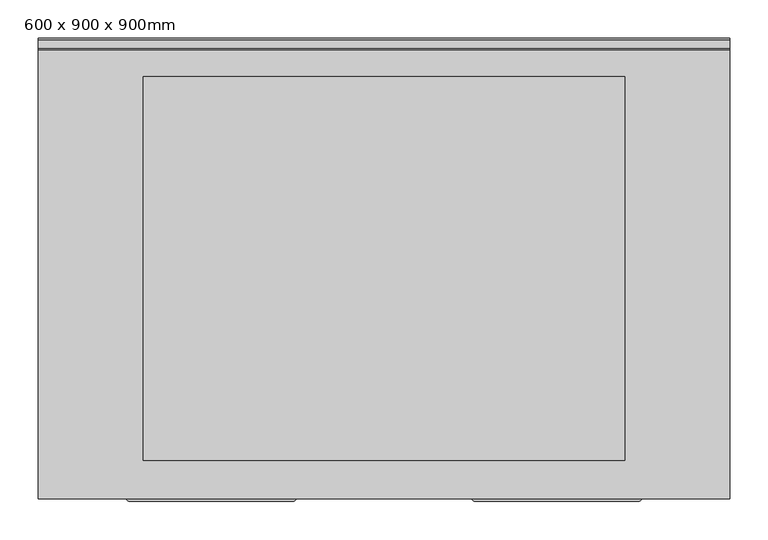
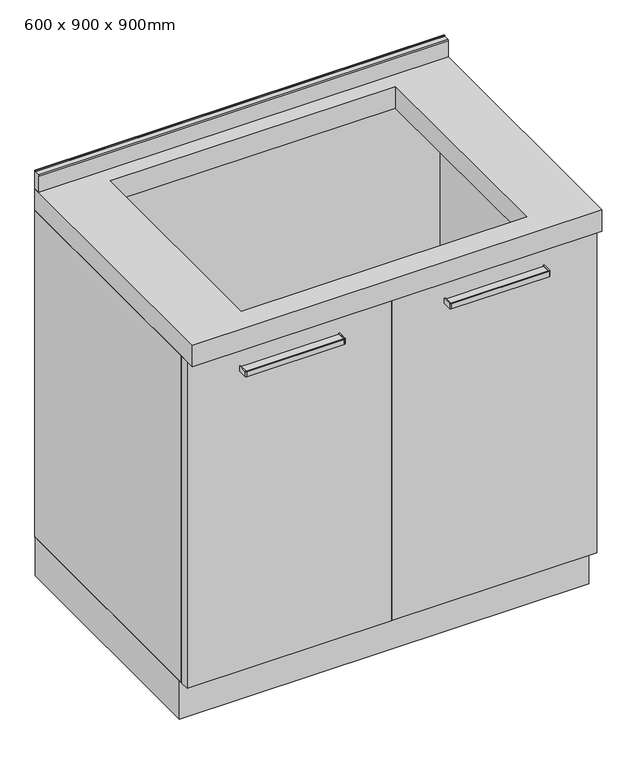
"""IFC4 building model written with IfcOpenShell, lengths in millimetres: furniture geometry, Küchenelement (1) - 2-flg - für Spüle : 600 x 900 x 900mm."""

import ifcopenshell
import ifcopenshell.guid

model = None  # the IFC model being written
_history = None  # IfcOwnerHistory: only IFC2X3 demands one
_inside = {}  # id of a spatial element -> (the spatial element, [elements in it])
_under = {}  # id of a project, library or spatial element -> (it, [spatial elements below it])
_declared = {}  # id of a project -> (the project, [libraries it declares])
_typed = {}  # id of a type object -> (the type object, [elements of that type])
_made_of = {}  # id of a material, layer set ... -> (it, [elements and type objects made of it])


def new_model(schema):
    """Start an empty IFC model of exactly this schema.

    Asked for "IFC4X3", IfcOpenShell would pick the latest addendum, in which some entities
    have other attributes; the version numbers below select the first issue.
    IFC2X3 requires an IfcOwnerHistory on every rooted entity: one is made here for all.
    """
    global model, _history
    if schema == "IFC4X3":
        model = ifcopenshell.file(schema_version=(4, 3, 0, 0))
    else:
        model = ifcopenshell.file(schema=schema)
    _inside.clear()
    _under.clear()
    _declared.clear()
    _typed.clear()
    _made_of.clear()
    _history = None
    if model.schema == "IFC2X3":
        org = make("IfcOrganization", Name="unknown")
        user = make(
            "IfcPersonAndOrganization",
            ThePerson=make("IfcPerson", FamilyName="unknown"),
            TheOrganization=org,
        )
        app = make(
            "IfcApplication",
            ApplicationDeveloper=org,
            Version="unknown",
            ApplicationFullName="unknown",
            ApplicationIdentifier="unknown",
        )
        _history = make(
            "IfcOwnerHistory",
            OwningUser=user,
            OwningApplication=app,
            ChangeAction="ADDED",
            CreationDate=0,
        )
    return model


def make(cls, **values):
    """One entity of the class cls with the attributes given. An attribute that is None is left unset."""
    return model.create_entity(
        cls, **{name: value for name, value in values.items() if value is not None}
    )


def rooted(cls, **values):
    """An entity with a GlobalId (a new one), such as an element, a storey or a relation."""
    return make(cls, GlobalId=ifcopenshell.guid.new(), OwnerHistory=_history, **values)


def si_unit(unit_type, name, prefix=None):
    """IfcSIUnit, for example si_unit("LENGTHUNIT", "METRE", prefix="MILLI")."""
    return make("IfcSIUnit", UnitType=unit_type, Prefix=prefix, Name=name)


def assignment(units):
    """IfcUnitAssignment: the units of a project."""
    return None if units is None else make("IfcUnitAssignment", Units=units)


def point(xyz):
    """IfcCartesianPoint."""
    return None if xyz is None else make("IfcCartesianPoint", Coordinates=xyz)


def direction(xyz):
    """IfcDirection."""
    return None if xyz is None else make("IfcDirection", DirectionRatios=xyz)


def frame(location, z_axis=None, x_axis=None):
    """IfcAxis2Placement3D, a coordinate frame: its origin and axes. An axis left out is left unset."""
    return make(
        "IfcAxis2Placement3D",
        Location=point(location),
        Axis=direction(z_axis),
        RefDirection=direction(x_axis),
    )


def frame_2d(location, x_axis=None):
    """IfcAxis2Placement2D, a coordinate frame in the plane: its origin and x axis."""
    return make(
        "IfcAxis2Placement2D", Location=point(location), RefDirection=direction(x_axis)
    )


def origin():
    """The frame at (0, 0, 0) with its axes left unset."""
    return frame((0.0, 0.0, 0.0))


def origin_with_axes():
    """The frame at (0, 0, 0) with the z axis (0, 0, 1) and the x axis (1, 0, 0) written out."""
    return frame((0.0, 0.0, 0.0), z_axis=(0.0, 0.0, 1.0), x_axis=(1.0, 0.0, 0.0))


def place(relative_to, where):
    """IfcLocalPlacement: puts the frame where relative to a parent placement (None: the world)."""
    return make(
        "IfcLocalPlacement", PlacementRelTo=relative_to, RelativePlacement=where
    )


def context(
    kind, dimensions, precision=None, world=None, true_north=None, identifier=None
):
    """IfcGeometricRepresentationContext, for example the 3D "Model" context."""
    return make(
        "IfcGeometricRepresentationContext",
        ContextIdentifier=identifier,
        ContextType=kind,
        CoordinateSpaceDimension=dimensions,
        Precision=precision,
        WorldCoordinateSystem=world,
        TrueNorth=true_north,
    )


def project(units=None, contexts=None):
    """IfcProject with its units and contexts."""
    return rooted(
        "IfcProject",
        Name="project",
        RepresentationContexts=contexts,
        UnitsInContext=assignment(units),
    )


def spatial(cls, under=None, at=None, **own):
    """A site, building, storey or space (cls), placed at a placement, below another one or the project."""
    s = rooted(cls, ObjectPlacement=at, **own)
    if under is not None:
        _under.setdefault(under.id(), (under, []))[1].append(s)
    return s


def polyline(points):
    """IfcPolyline through the points."""
    return make("IfcPolyline", Points=[point(p) for p in points])


def circle_curve(where, radius):
    """IfcCircle in the frame where."""
    return make("IfcCircle", Position=where, Radius=radius)


def trimmed(basis, trim1, trim2, sense, master):
    """IfcTrimmedCurve: the piece of a basis curve between two trims."""
    return make(
        "IfcTrimmedCurve",
        BasisCurve=basis,
        Trim1=trim1,
        Trim2=trim2,
        SenseAgreement=sense,
        MasterRepresentation=master,
    )


def segment(curve, same_sense, transition):
    """IfcCompositeCurveSegment."""
    return make(
        "IfcCompositeCurveSegment",
        Transition=transition,
        SameSense=same_sense,
        ParentCurve=curve,
    )


def composite_curve(segments, self_intersect=None):
    """IfcCompositeCurve: segments joined end to end."""
    return make("IfcCompositeCurve", Segments=segments, SelfIntersect=self_intersect)


def outline(outer, holes=None, kind="AREA"):
    """IfcArbitraryClosedProfileDef: a profile drawn as a closed curve; with holes, ...WithVoids."""
    if holes is None:
        return make("IfcArbitraryClosedProfileDef", ProfileType=kind, OuterCurve=outer)
    return make(
        "IfcArbitraryProfileDefWithVoids",
        ProfileType=kind,
        OuterCurve=outer,
        InnerCurves=holes,
    )


def extrude(swept, where, along, depth):
    """IfcExtrudedAreaSolid: the profile swept, set in the frame where, extruded along a direction by depth."""
    return make(
        "IfcExtrudedAreaSolid",
        SweptArea=swept,
        Position=where,
        ExtrudedDirection=direction(along),
        Depth=depth,
    )


def shape(context_of_items, identifier, shape_type, items):
    """IfcShapeRepresentation: the items that make up one representation, for example the "Body"."""
    return make(
        "IfcShapeRepresentation",
        ContextOfItems=context_of_items,
        RepresentationIdentifier=identifier,
        RepresentationType=shape_type,
        Items=items,
    )


def source(mapping_origin, context_of_items, identifier, shape_type, items):
    """IfcRepresentationMap: a shape defined once, which mapped items show again and again."""
    return make(
        "IfcRepresentationMap",
        MappingOrigin=mapping_origin,
        MappedRepresentation=shape(context_of_items, identifier, shape_type, items),
    )


def transform(
    local_origin,
    x_axis=None,
    y_axis=None,
    z_axis=None,
    scale=None,
    scale2=None,
    scale3=None,
    uniform=True,
):
    """IfcCartesianTransformationOperator3D, or its non-uniform kind. x_axis, y_axis, z_axis: its Axis1, 2, 3."""
    if uniform:
        return make(
            "IfcCartesianTransformationOperator3D",
            Axis1=direction(x_axis),
            Axis2=direction(y_axis),
            LocalOrigin=point(local_origin),
            Scale=scale,
            Axis3=direction(z_axis),
        )
    return make(
        "IfcCartesianTransformationOperator3DnonUniform",
        Axis1=direction(x_axis),
        Axis2=direction(y_axis),
        LocalOrigin=point(local_origin),
        Scale=scale,
        Axis3=direction(z_axis),
        Scale2=scale2,
        Scale3=scale3,
    )


def mapped(mapping_source, mapping_target):
    """IfcMappedItem: shows the shape of a source again, moved by a transform."""
    return make(
        "IfcMappedItem", MappingSource=mapping_source, MappingTarget=mapping_target
    )


def made_of(thing, what):
    """Note that an element or type object is made of a material, layer set ...; save() writes the relation."""
    if what is not None:
        _made_of.setdefault(what.id(), (what, []))[1].append(thing)
    return thing


def element(
    cls,
    number,
    at=None,
    inside=None,
    cuts=None,
    type_object=None,
    material=None,
    context=None,
    identifier="Body",
    shape_type=None,
    held_by="IfcProductDefinitionShape",
    body=None,
    shapes=None,
    **own,
):
    """One element of the class cls, such as IfcWall. Its Tag is "e" and its number.

    at: its placement. inside: the storey or other place that contains it. cuts: it is an
    opening in that element (IfcRelVoidsElement). A single representation is given by context,
    identifier, shape_type and body (its items); several are given by shapes. held_by: the class
    of the entity that holds the representations. save() writes the other relations.
    """
    e = rooted(cls, Tag="e%d" % number, ObjectPlacement=at, **own)
    if body is not None:
        shapes = [shape(context, identifier, shape_type, body)]
    if shapes is not None:
        e.Representation = make(held_by, Representations=shapes)
    if inside is not None:
        _inside.setdefault(inside.id(), (inside, []))[1].append(e)
    if cuts is not None:
        rooted(
            "IfcRelVoidsElement", RelatingBuildingElement=cuts, RelatedOpeningElement=e
        )
    if type_object is not None:
        _typed.setdefault(type_object.id(), (type_object, []))[1].append(e)
    return made_of(e, material)


def aggregate(whole, parts):
    """IfcRelAggregates: a whole, such as a stair, and the parts it consists of."""
    return rooted("IfcRelAggregates", RelatingObject=whole, RelatedObjects=parts)


def save(model, path):
    """Write the relations noted so far, then the file.

    IfcRelAggregates (storeys below a building ...), IfcRelContainedInSpatialStructure (elements
    in a storey), IfcRelDefinesByType, IfcRelAssociatesMaterial and IfcRelDeclares: one each for
    every whole, place, type object, material and project.
    """
    for whole, parts in _under.values():
        aggregate(whole, parts)
    for where, things in _inside.values():
        rooted(
            "IfcRelContainedInSpatialStructure",
            RelatedElements=things,
            RelatingStructure=where,
        )
    for kind, things in _typed.values():
        rooted("IfcRelDefinesByType", RelatedObjects=things, RelatingType=kind)
    for what, things in _made_of.values():
        rooted("IfcRelAssociatesMaterial", RelatedObjects=things, RelatingMaterial=what)
    for by, libraries in _declared.values():
        rooted("IfcRelDeclares", RelatingContext=by, RelatedDefinitions=libraries)
    model.write(path)


def furniture_600_x_900_x_900mm_7960ee9d(model_context):
    return source(origin(), model_context, "Body", "SweptSolid", [
        extrude(outline(composite_curve([segment(polyline([(161.7003264, -580.0), (377.7003264, -580.0), (377.7003264, -600.5)]), True, "CONTINUOUS"), segment(trimmed(circle_curve(frame_2d((377.2003264, -600.5)), 0.5), [point((377.7003264, -600.5))], [point((377.2003264, -601.0))], False, "CARTESIAN"), True, "CONTINUOUS"), segment(polyline([(377.2003264, -601.0), (162.2003264, -601.0)]), True, "CONTINUOUS"), segment(trimmed(circle_curve(frame_2d((162.2003264, -600.5)), 0.5), [point((162.2003264, -601.0))], [point((161.7003264, -600.5))], False, "CARTESIAN"), True, "CONTINUOUS"), segment(polyline([(161.7003264, -600.5), (161.7003264, -580.0)]), True, "CONTINUOUS")], self_intersect=False)), frame((0.0, 0.0, 789.965389), z_axis=(0.0, 0.0, 1.0), x_axis=(1.0, 0.0, 0.0)), (0.0, 0.0, 1.0), 6.4890959),
        extrude(outline(composite_curve([segment(polyline([(159.7003264, -580.0), (161.7003264, -580.0), (161.7003264, -600.5)]), True, "CONTINUOUS"), segment(trimmed(circle_curve(frame_2d((162.2003264, -600.5)), 0.5), [point((161.7003264, -600.5))], [point((162.2003264, -601.0))], True, "CARTESIAN"), True, "CONTINUOUS"), segment(polyline([(162.2003264, -601.0), (377.2003264, -601.0)]), True, "CONTINUOUS"), segment(trimmed(circle_curve(frame_2d((377.2003264, -600.5)), 0.5), [point((377.2003264, -601.0))], [point((377.7003264, -600.5))], True, "CARTESIAN"), True, "CONTINUOUS"), segment(polyline([(377.7003264, -600.5), (377.7003264, -580.0), (379.7003264, -580.0), (379.7003264, -600.5)]), True, "CONTINUOUS"), segment(trimmed(circle_curve(frame_2d((377.2003264, -600.5)), 2.5), [point((379.7003264, -600.5))], [point((377.2003264, -603.0))], False, "CARTESIAN"), True, "CONTINUOUS"), segment(polyline([(377.2003264, -603.0), (162.2003264, -603.0)]), True, "CONTINUOUS"), segment(trimmed(circle_curve(frame_2d((162.2003264, -600.5)), 2.5), [point((162.2003264, -603.0))], [point((159.7003264, -600.5))], False, "CARTESIAN"), True, "CONTINUOUS"), segment(polyline([(159.7003264, -600.5), (159.7003264, -580.0)]), True, "CONTINUOUS")], self_intersect=False)), frame((0.0, 0.0, 787.2), z_axis=(0.0, 0.0, 1.0), x_axis=(1.0, 0.0, 0.0)), (0.0, 0.0, 1.0), 12.0),
        extrude(outline(composite_curve([segment(polyline([(-288.2996736, -580.0), (-72.2996736, -580.0), (-72.2996736, -600.5)]), True, "CONTINUOUS"), segment(trimmed(circle_curve(frame_2d((-72.7996736, -600.5)), 0.5), [point((-72.2996736, -600.5))], [point((-72.7996736, -601.0))], False, "CARTESIAN"), True, "CONTINUOUS"), segment(polyline([(-72.7996736, -601.0), (-287.7996736, -601.0)]), True, "CONTINUOUS"), segment(trimmed(circle_curve(frame_2d((-287.7996736, -600.5)), 0.5), [point((-287.7996736, -601.0))], [point((-288.2996736, -600.5))], False, "CARTESIAN"), True, "CONTINUOUS"), segment(polyline([(-288.2996736, -600.5), (-288.2996736, -580.0)]), True, "CONTINUOUS")], self_intersect=False)), frame((0.0, 0.0, 789.965389), z_axis=(0.0, 0.0, 1.0), x_axis=(1.0, 0.0, 0.0)), (0.0, 0.0, 1.0), 6.4890959),
        extrude(outline(composite_curve([segment(polyline([(-290.2996736, -580.0), (-288.2996736, -580.0), (-288.2996736, -600.5)]), True, "CONTINUOUS"), segment(trimmed(circle_curve(frame_2d((-287.7996736, -600.5)), 0.5), [point((-288.2996736, -600.5))], [point((-287.7996736, -601.0))], True, "CARTESIAN"), True, "CONTINUOUS"), segment(polyline([(-287.7996736, -601.0), (-72.7996736, -601.0)]), True, "CONTINUOUS"), segment(trimmed(circle_curve(frame_2d((-72.7996736, -600.5)), 0.5), [point((-72.7996736, -601.0))], [point((-72.2996736, -600.5))], True, "CARTESIAN"), True, "CONTINUOUS"), segment(polyline([(-72.2996736, -600.5), (-72.2996736, -580.0), (-70.2996736, -580.0), (-70.2996736, -600.5)]), True, "CONTINUOUS"), segment(trimmed(circle_curve(frame_2d((-72.7996736, -600.5)), 2.5), [point((-70.2996736, -600.5))], [point((-72.7996736, -603.0))], False, "CARTESIAN"), True, "CONTINUOUS"), segment(polyline([(-72.7996736, -603.0), (-287.7996736, -603.0)]), True, "CONTINUOUS"), segment(trimmed(circle_curve(frame_2d((-287.7996736, -600.5)), 2.5), [point((-287.7996736, -603.0))], [point((-290.2996736, -600.5))], False, "CARTESIAN"), True, "CONTINUOUS"), segment(polyline([(-290.2996736, -600.5), (-290.2996736, -580.0)]), True, "CONTINUOUS")], self_intersect=False)), frame((0.0, 0.0, 787.2), z_axis=(0.0, 0.0, 1.0), x_axis=(1.0, 0.0, 0.0)), (0.0, 0.0, 1.0), 12.0),
        extrude(outline(composite_curve([segment(polyline([(0.0, 942.0034681), (0.0, 900.0), (-15.0, 900.0), (-15.0, 938.0)]), True, "CONTINUOUS"), segment(trimmed(circle_curve(frame_2d((-13.0, 938.0)), 2.0), [point((-15.0, 938.0))], [point((-13.0, 940.0))], False, "CARTESIAN"), True, "CONTINUOUS"), segment(polyline([(-13.0, 940.0), (-1.50449, 940.0), (-1.50449, 942.0034681), (0.0, 942.0034681)]), True, "CONTINUOUS")], self_intersect=False)), frame((-405.2996736, 0.0, 0.0), z_axis=(1.0, 0.0, 0.0), x_axis=(0.0, 1.0, 0.0)), (0.0, 0.0, 1.0), 900.0),
        extrude(outline(polyline([(494.7003264, -0.533703), (494.7003264, -550.533703), (-405.2996736, -550.533703), (-405.2996736, -0.533703), (494.7003264, -0.533703)])), origin_with_axes(), (0.0, 0.0, 1.0), 90.0),
        extrude(outline(polyline([(494.7003264, 0.0), (494.7003264, -600.0), (-405.2996736, -600.0), (-405.2996736, 0.0), (494.7003264, 0.0)]), holes=[polyline([(358.2003264, -49.8), (-268.7996736, -49.8), (-268.7996736, -549.8), (358.2003264, -549.8), (358.2003264, -49.8)])]), frame((0.0, 0.0, 850.0), z_axis=(0.0, 0.0, 1.0), x_axis=(1.0, 0.0, 0.0)), (0.0, 0.0, 1.0), 50.0),
        extrude(outline(polyline([(43.7003264, -580.0), (-405.2996736, -580.0), (-405.2996736, -558.0), (43.7003264, -558.0), (43.7003264, -580.0)])), frame((0.0, 0.0, 90.0), z_axis=(0.0, 0.0, 1.0), x_axis=(1.0, 0.0, 0.0)), (0.0, 0.0, 1.0), 760.0),
        extrude(outline(polyline([(45.7003264, -580.0), (45.7003264, -558.0), (494.7003264, -558.0), (494.7003264, -580.0), (45.7003264, -580.0)])), frame((0.0, 0.0, 90.0), z_axis=(0.0, 0.0, 1.0), x_axis=(1.0, 0.0, 0.0)), (0.0, 0.0, 1.0), 760.0),
        extrude(outline(polyline([(494.7003264, 0.0), (494.7003264, -558.0), (472.7003264, -558.0), (472.7003264, -22.0), (-383.2996736, -22.0), (-383.2996736, -558.0), (-405.2996736, -558.0), (-405.2996736, 0.0), (494.7003264, 0.0)])), frame((0.0, 0.0, 90.0), z_axis=(0.0, 0.0, 1.0), x_axis=(1.0, 0.0, 0.0)), (0.0, 0.0, 1.0), 760.0),
    ])


if __name__ == "__main__":
    model = new_model("IFC4")
    model_context = context("Model", 3, world=origin())
    ifc_project = project(units=[si_unit("LENGTHUNIT", "METRE", prefix="MILLI")], contexts=[model_context])
    site = spatial("IfcSite", under=ifc_project)
    building = spatial("IfcBuilding", under=site)
    placement = place(None, origin())
    furniture_600_x_900_x_900mm_shape = furniture_600_x_900_x_900mm_7960ee9d(model_context)
    element("IfcFurniture", 1, ObjectType="Küchenelement (1) - 2-flg - für Spüle : 600 x 900 x 900mm", at=placement, inside=building, context=model_context, shape_type="MappedRepresentation", body=[
        mapped(furniture_600_x_900_x_900mm_shape, transform((0.0, 0.0, 0.0), x_axis=(1.0, 0.0, 0.0), y_axis=(0.0, 1.0, 0.0), z_axis=(0.0, 0.0, 1.0))),
    ])
    save(model, "model.ifc")

# Revit data of these elements
# Type "Küchenelement (1) - 2-flg - für Spüle : 600 x 900 x 900mm"
#   Assembly Code = "C1030400"
#   Länge 1 = 0.1008 m
#   Depth = 0.600 m
#   Height = 0.900 m
#   Width = 0.900 m
#   Obermaterial = none
#   Material = none
#   Griffmaterial = none
# Element 1 (IfcFurniture, "Küchenelement (1) - 2-flg - für Spüle : 600 x 900 x 900mm")
#   Materials on its faces: "Holz - Birke"
# Materials
#   "Holz - Birke": class "Holz", colour RGB 213 164 103, transparency 0, Cost = 0
